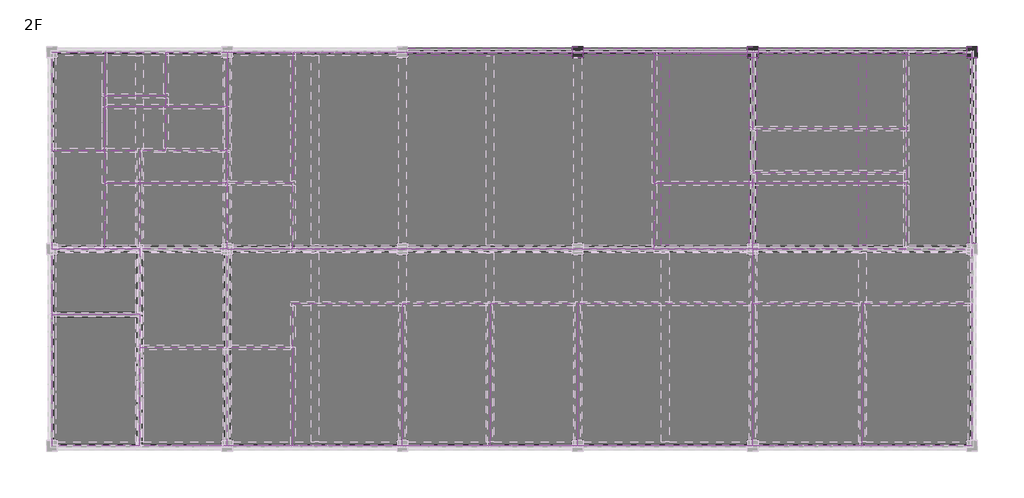
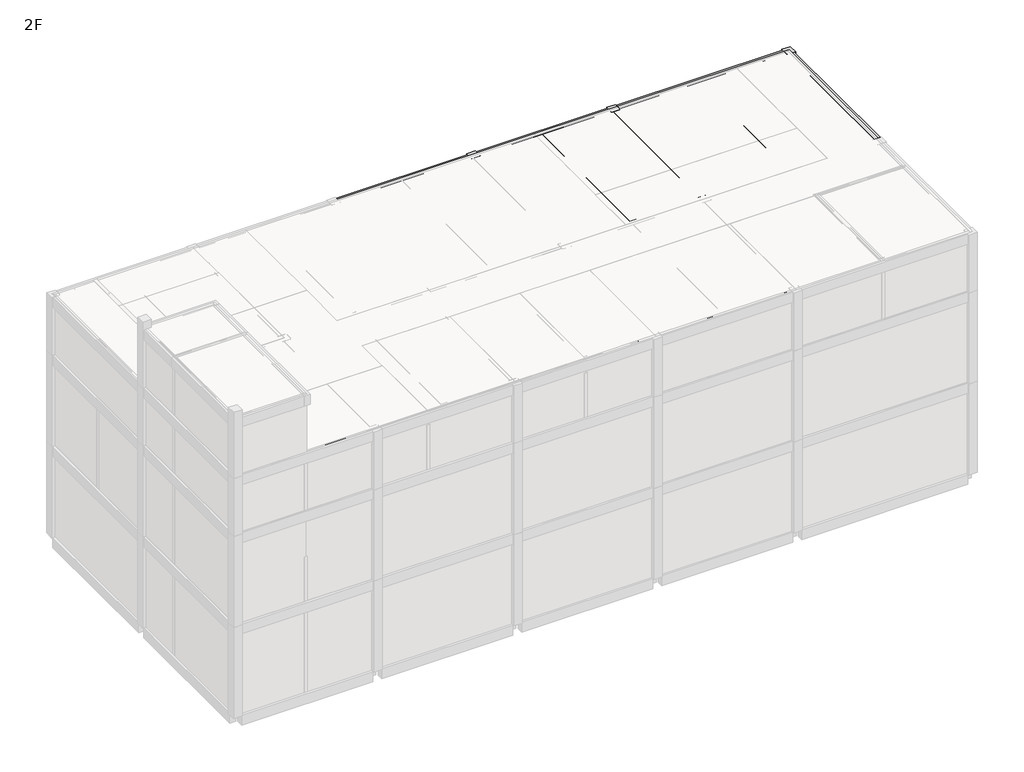
# One storey, part 7 of 7: 39 proxies, 28 beams, 9 columns.
"""IFC4 building model written with IfcOpenShell, lengths in millimetres."""

import ifcopenshell
import ifcopenshell.guid

model = None  # the IFC model being written
_history = None  # IfcOwnerHistory: only IFC2X3 demands one
_inside = {}  # id of a spatial element -> (the spatial element, [elements in it])
_under = {}  # id of a project, library or spatial element -> (it, [spatial elements below it])
_declared = {}  # id of a project -> (the project, [libraries it declares])
_typed = {}  # id of a type object -> (the type object, [elements of that type])
_made_of = {}  # id of a material, layer set ... -> (it, [elements and type objects made of it])


def new_model(schema):
    """Start an empty IFC model of exactly this schema.

    Asked for "IFC4X3", IfcOpenShell would pick the latest addendum, in which some entities
    have other attributes; the version numbers below select the first issue.
    IFC2X3 requires an IfcOwnerHistory on every rooted entity: one is made here for all.
    """
    global model, _history
    if schema == "IFC4X3":
        model = ifcopenshell.file(schema_version=(4, 3, 0, 0))
    else:
        model = ifcopenshell.file(schema=schema)
    _inside.clear()
    _under.clear()
    _declared.clear()
    _typed.clear()
    _made_of.clear()
    _history = None
    if model.schema == "IFC2X3":
        org = make("IfcOrganization", Name="unknown")
        user = make(
            "IfcPersonAndOrganization",
            ThePerson=make("IfcPerson", FamilyName="unknown"),
            TheOrganization=org,
        )
        app = make(
            "IfcApplication",
            ApplicationDeveloper=org,
            Version="unknown",
            ApplicationFullName="unknown",
            ApplicationIdentifier="unknown",
        )
        _history = make(
            "IfcOwnerHistory",
            OwningUser=user,
            OwningApplication=app,
            ChangeAction="ADDED",
            CreationDate=0,
        )
    return model


def make(cls, **values):
    """One entity of the class cls with the attributes given. An attribute that is None is left unset."""
    return model.create_entity(
        cls, **{name: value for name, value in values.items() if value is not None}
    )


def rooted(cls, **values):
    """An entity with a GlobalId (a new one), such as an element, a storey or a relation."""
    return make(cls, GlobalId=ifcopenshell.guid.new(), OwnerHistory=_history, **values)


def si_unit(unit_type, name, prefix=None):
    """IfcSIUnit, for example si_unit("LENGTHUNIT", "METRE", prefix="MILLI")."""
    return make("IfcSIUnit", UnitType=unit_type, Prefix=prefix, Name=name)


def assignment(units):
    """IfcUnitAssignment: the units of a project."""
    return None if units is None else make("IfcUnitAssignment", Units=units)


def point(xyz):
    """IfcCartesianPoint."""
    return None if xyz is None else make("IfcCartesianPoint", Coordinates=xyz)


def direction(xyz):
    """IfcDirection."""
    return None if xyz is None else make("IfcDirection", DirectionRatios=xyz)


def frame(location, z_axis=None, x_axis=None):
    """IfcAxis2Placement3D, a coordinate frame: its origin and axes. An axis left out is left unset."""
    return make(
        "IfcAxis2Placement3D",
        Location=point(location),
        Axis=direction(z_axis),
        RefDirection=direction(x_axis),
    )


def origin():
    """The frame at (0, 0, 0) with its axes left unset."""
    return frame((0.0, 0.0, 0.0))


def origin_with_axes():
    """The frame at (0, 0, 0) with the z axis (0, 0, 1) and the x axis (1, 0, 0) written out."""
    return frame((0.0, 0.0, 0.0), z_axis=(0.0, 0.0, 1.0), x_axis=(1.0, 0.0, 0.0))


def place(relative_to, where):
    """IfcLocalPlacement: puts the frame where relative to a parent placement (None: the world)."""
    return make(
        "IfcLocalPlacement", PlacementRelTo=relative_to, RelativePlacement=where
    )


def context(
    kind, dimensions, precision=None, world=None, true_north=None, identifier=None
):
    """IfcGeometricRepresentationContext, for example the 3D "Model" context."""
    return make(
        "IfcGeometricRepresentationContext",
        ContextIdentifier=identifier,
        ContextType=kind,
        CoordinateSpaceDimension=dimensions,
        Precision=precision,
        WorldCoordinateSystem=world,
        TrueNorth=true_north,
    )


def project(units=None, contexts=None):
    """IfcProject with its units and contexts."""
    return rooted(
        "IfcProject",
        Name="project",
        RepresentationContexts=contexts,
        UnitsInContext=assignment(units),
    )


def spatial(cls, under=None, at=None, **own):
    """A site, building, storey or space (cls), placed at a placement, below another one or the project."""
    s = rooted(cls, ObjectPlacement=at, **own)
    if under is not None:
        _under.setdefault(under.id(), (under, []))[1].append(s)
    return s


def polyline(points):
    """IfcPolyline through the points."""
    return make("IfcPolyline", Points=[point(p) for p in points])


def outline(outer, holes=None, kind="AREA"):
    """IfcArbitraryClosedProfileDef: a profile drawn as a closed curve; with holes, ...WithVoids."""
    if holes is None:
        return make("IfcArbitraryClosedProfileDef", ProfileType=kind, OuterCurve=outer)
    return make(
        "IfcArbitraryProfileDefWithVoids",
        ProfileType=kind,
        OuterCurve=outer,
        InnerCurves=holes,
    )


def extrude(swept, where, along, depth):
    """IfcExtrudedAreaSolid: the profile swept, set in the frame where, extruded along a direction by depth."""
    return make(
        "IfcExtrudedAreaSolid",
        SweptArea=swept,
        Position=where,
        ExtrudedDirection=direction(along),
        Depth=depth,
    )


def faces_of(points, faces, orient=None, outer=None):
    """IfcFace entities. A face is a list of loops; a loop is a list of indices into points, from 0.

    orient and outer hold one flag for each loop. By default every Orientation is true, the
    first loop of a face is its IfcFaceOuterBound and the others are IfcFaceBound.
    """
    made = []
    for i, loops in enumerate(faces):
        bounds = []
        for j, loop in enumerate(loops):
            is_outer = j == 0 if outer is None else outer[i][j]
            bounds.append(
                make(
                    "IfcFaceOuterBound" if is_outer else "IfcFaceBound",
                    Bound=make("IfcPolyLoop", Polygon=[points[k] for k in loop]),
                    Orientation=True if orient is None else orient[i][j],
                )
            )
        made.append(make("IfcFace", Bounds=bounds))
    return made


def faceted_brep(points, faces, orient=None, outer=None, voids=None):
    """IfcFacetedBrep: a solid bounded by flat faces; with voids (closed shells), ...WithVoids."""
    shared = [point(p) for p in points]
    hull = make("IfcClosedShell", CfsFaces=faces_of(shared, faces, orient, outer))
    if voids is None:
        return make("IfcFacetedBrep", Outer=hull)
    return make(
        "IfcFacetedBrepWithVoids",
        Outer=hull,
        Voids=[
            make(cls, CfsFaces=faces_of(shared, fs, o, b)) for cls, fs, o, b in voids
        ],
    )


def shape(context_of_items, identifier, shape_type, items):
    """IfcShapeRepresentation: the items that make up one representation, for example the "Body"."""
    return make(
        "IfcShapeRepresentation",
        ContextOfItems=context_of_items,
        RepresentationIdentifier=identifier,
        RepresentationType=shape_type,
        Items=items,
    )


def source(mapping_origin, context_of_items, identifier, shape_type, items):
    """IfcRepresentationMap: a shape defined once, which mapped items show again and again."""
    return make(
        "IfcRepresentationMap",
        MappingOrigin=mapping_origin,
        MappedRepresentation=shape(context_of_items, identifier, shape_type, items),
    )


def transform(
    local_origin,
    x_axis=None,
    y_axis=None,
    z_axis=None,
    scale=None,
    scale2=None,
    scale3=None,
    uniform=True,
):
    """IfcCartesianTransformationOperator3D, or its non-uniform kind. x_axis, y_axis, z_axis: its Axis1, 2, 3."""
    if uniform:
        return make(
            "IfcCartesianTransformationOperator3D",
            Axis1=direction(x_axis),
            Axis2=direction(y_axis),
            LocalOrigin=point(local_origin),
            Scale=scale,
            Axis3=direction(z_axis),
        )
    return make(
        "IfcCartesianTransformationOperator3DnonUniform",
        Axis1=direction(x_axis),
        Axis2=direction(y_axis),
        LocalOrigin=point(local_origin),
        Scale=scale,
        Axis3=direction(z_axis),
        Scale2=scale2,
        Scale3=scale3,
    )


def mapped(mapping_source, mapping_target):
    """IfcMappedItem: shows the shape of a source again, moved by a transform."""
    return make(
        "IfcMappedItem", MappingSource=mapping_source, MappingTarget=mapping_target
    )


def made_of(thing, what):
    """Note that an element or type object is made of a material, layer set ...; save() writes the relation."""
    if what is not None:
        _made_of.setdefault(what.id(), (what, []))[1].append(thing)
    return thing


def element(
    cls,
    number,
    at=None,
    inside=None,
    cuts=None,
    type_object=None,
    material=None,
    context=None,
    identifier="Body",
    shape_type=None,
    held_by="IfcProductDefinitionShape",
    body=None,
    shapes=None,
    **own,
):
    """One element of the class cls, such as IfcWall. Its Tag is "e" and its number.

    at: its placement. inside: the storey or other place that contains it. cuts: it is an
    opening in that element (IfcRelVoidsElement). A single representation is given by context,
    identifier, shape_type and body (its items); several are given by shapes. held_by: the class
    of the entity that holds the representations. save() writes the other relations.
    """
    e = rooted(cls, Tag="e%d" % number, ObjectPlacement=at, **own)
    if body is not None:
        shapes = [shape(context, identifier, shape_type, body)]
    if shapes is not None:
        e.Representation = make(held_by, Representations=shapes)
    if inside is not None:
        _inside.setdefault(inside.id(), (inside, []))[1].append(e)
    if cuts is not None:
        rooted(
            "IfcRelVoidsElement", RelatingBuildingElement=cuts, RelatedOpeningElement=e
        )
    if type_object is not None:
        _typed.setdefault(type_object.id(), (type_object, []))[1].append(e)
    return made_of(e, material)


def aggregate(whole, parts):
    """IfcRelAggregates: a whole, such as a stair, and the parts it consists of."""
    return rooted("IfcRelAggregates", RelatingObject=whole, RelatedObjects=parts)


def save(model, path):
    """Write the relations noted so far, then the file.

    IfcRelAggregates (storeys below a building ...), IfcRelContainedInSpatialStructure (elements
    in a storey), IfcRelDefinesByType, IfcRelAssociatesMaterial and IfcRelDeclares: one each for
    every whole, place, type object, material and project.
    """
    for whole, parts in _under.values():
        aggregate(whole, parts)
    for where, things in _inside.values():
        rooted(
            "IfcRelContainedInSpatialStructure",
            RelatedElements=things,
            RelatingStructure=where,
        )
    for kind, things in _typed.values():
        rooted("IfcRelDefinesByType", RelatedObjects=things, RelatingType=kind)
    for what, things in _made_of.values():
        rooted("IfcRelAssociatesMaterial", RelatedObjects=things, RelatingMaterial=what)
    for by, libraries in _declared.values():
        rooted("IfcRelDeclares", RelatingContext=by, RelatedDefinitions=libraries)
    model.write(path)


def generic_models_c89eb543(model_context):
    return source(origin(), model_context, "Body", "SweptSolid", [
        extrude(outline(polyline([(2000.0, 3000.0), (2000.0, -3000.0), (-2000.0, -3000.0), (-2000.0, 3000.0), (2000.0, 3000.0)])), origin_with_axes(), (0.0, 0.0, 1.0), 3500.0),
    ])


def generic_models_50f5a469(model_context):
    return source(origin(), model_context, "Body", "SweptSolid", [
        extrude(outline(polyline([(4500.0, 16000.0), (4500.0, -16000.0), (-4500.0, -16000.0), (-4500.0, 16000.0), (4500.0, 16000.0)])), origin_with_axes(), (0.0, 0.0, 1.0), 5500.0),
    ])


def generic_models_8b5775ea(model_context):
    return source(origin(), model_context, "Body", "SweptSolid", [
        extrude(outline(polyline([(4500.0, 17000.0), (4500.0, -17000.0), (-4500.0, -17000.0), (-4500.0, 17000.0), (4500.0, 17000.0)])), origin_with_axes(), (0.0, 0.0, 1.0), 5500.0),
    ])


def generic_models_2d265e4a(model_context):
    return source(origin(), model_context, "Body", "SweptSolid", [
        extrude(outline(polyline([(4500.0, 5000.0), (4500.0, -5000.0), (-4500.0, -5000.0), (-4500.0, 5000.0), (4500.0, 5000.0)])), origin_with_axes(), (0.0, 0.0, 1.0), 5500.0),
    ])


def generic_models_8934d72c(model_context):
    return source(origin(), model_context, "Body", "SweptSolid", [
        extrude(outline(polyline([(2000.0, 4500.0), (2000.0, -4500.0), (-2000.0, -4500.0), (-2000.0, 4500.0), (2000.0, 4500.0)])), origin_with_axes(), (0.0, 0.0, 1.0), 5500.0),
    ])


def generic_models_626d8198(model_context):
    return source(origin(), model_context, "Body", "SweptSolid", [
        extrude(outline(polyline([(2000.0, 1500.0), (2000.0, -1500.0), (-2000.0, -1500.0), (-2000.0, 1500.0), (2000.0, 1500.0)])), origin_with_axes(), (0.0, 0.0, 1.0), 5500.0),
    ])


def generic_models_cc1dae17(model_context):
    return source(origin(), model_context, "Body", "SweptSolid", [
        extrude(outline(polyline([(2000.0, 3000.0), (2000.0, -3000.0), (-2000.0, -3000.0), (-2000.0, 3000.0), (2000.0, 3000.0)])), origin_with_axes(), (0.0, 0.0, 1.0), 5500.0),
    ])


def generic_models_7ea3b148(model_context):
    return source(origin(), model_context, "Body", "SweptSolid", [
        extrude(outline(polyline([(4500.0, 12000.0), (4500.0, -12000.0), (-4500.0, -12000.0), (-4500.0, 12000.0), (4500.0, 12000.0)])), origin_with_axes(), (0.0, 0.0, 1.0), 5500.0),
    ])


def generic_models_85ff21bb(model_context):
    return source(origin(), model_context, "Body", "SweptSolid", [
        extrude(outline(polyline([(3500.0, 1750.0), (3500.0, -1750.0), (-3500.0, -1750.0), (-3500.0, 1750.0), (3500.0, 1750.0)])), origin_with_axes(), (0.0, 0.0, 1.0), 5500.0),
    ])


def generic_models_570012e4(model_context):
    return source(origin(), model_context, "Body", "SweptSolid", [
        extrude(outline(polyline([(1200.0, 2250.0), (1200.0, -2250.0), (-1200.0, -2250.0), (-1200.0, 2250.0), (1200.0, 2250.0)])), origin_with_axes(), (0.0, 0.0, 1.0), 5500.0),
    ])


def generic_models_971c0b89(model_context):
    return source(origin(), model_context, "Body", "SweptSolid", [
        extrude(outline(polyline([(2000.0, 2250.0), (2000.0, -2250.0), (-2000.0, -2250.0), (-2000.0, 2250.0), (2000.0, 2250.0)])), origin_with_axes(), (0.0, 0.0, 1.0), 5500.0),
    ])


def generic_models_ac48a1a3(model_context):
    return source(origin(), model_context, "Body", "SweptSolid", [
        extrude(outline(polyline([(1400.0, 2250.0), (1400.0, -2250.0), (-1400.0, -2250.0), (-1400.0, 2250.0), (1400.0, 2250.0)])), origin_with_axes(), (0.0, 0.0, 1.0), 5500.0),
    ])


def generic_models_ee32b0c6(model_context):
    return source(origin(), model_context, "Body", "SweptSolid", [
        extrude(outline(polyline([(1400.0, 1000.0), (1400.0, -1000.0), (-1400.0, -1000.0), (-1400.0, 1000.0), (1400.0, 1000.0)])), origin_with_axes(), (0.0, 0.0, 1.0), 5500.0),
    ])


def generic_models_0ee3397c(model_context):
    return source(origin(), model_context, "Body", "SweptSolid", [
        extrude(outline(polyline([(1400.0, 1250.0), (1400.0, -1250.0), (-1400.0, -1250.0), (-1400.0, 1250.0), (1400.0, 1250.0)])), origin_with_axes(), (0.0, 0.0, 1.0), 5500.0),
    ])


def generic_models_8c4134a9(model_context):
    return source(origin(), model_context, "Body", "SweptSolid", [
        extrude(outline(polyline([(3250.0, 2000.0), (3250.0, -2000.0), (-3250.0, -2000.0), (-3250.0, 2000.0), (3250.0, 2000.0)])), origin_with_axes(), (0.0, 0.0, 1.0), 3500.0),
    ])


def generic_models_ccc8c8c2(model_context):
    return source(origin(), model_context, "Body", "SweptSolid", [
        extrude(outline(polyline([(3000.0, 5750.0), (3000.0, -5750.0), (-3000.0, -5750.0), (-3000.0, 5750.0), (3000.0, 5750.0)])), origin_with_axes(), (0.0, 0.0, 1.0), 3500.0),
    ])


def generic_models_70f6ae48(model_context):
    return source(origin(), model_context, "Body", "SweptSolid", [
        extrude(outline(polyline([(3250.0, 4000.0), (3250.0, -4000.0), (-3250.0, -4000.0), (-3250.0, 4000.0), (3250.0, 4000.0)])), origin_with_axes(), (0.0, 0.0, 1.0), 3500.0),
    ])


def generic_models_f0561c1d(model_context):
    return source(origin(), model_context, "Body", "SweptSolid", [
        extrude(outline(polyline([(4500.0, 8250.0), (4500.0, -8250.0), (-4500.0, -8250.0), (-4500.0, 8250.0), (4500.0, 8250.0)])), origin_with_axes(), (0.0, 0.0, 1.0), 3500.0),
    ])


def generic_models_249c6621(model_context):
    return source(origin(), model_context, "Body", "SweptSolid", [
        extrude(outline(polyline([(3250.0, 2500.0), (3250.0, -2500.0), (-3250.0, -2500.0), (-3250.0, 2500.0), (3250.0, 2500.0)])), origin_with_axes(), (0.0, 0.0, 1.0), 3500.0),
    ])


def generic_models_f1f4091a(model_context):
    return source(origin(), model_context, "Body", "SweptSolid", [
        extrude(outline(polyline([(1500.0, 5750.0), (1500.0, -5750.0), (-1500.0, -5750.0), (-1500.0, 5750.0), (1500.0, 5750.0)])), origin_with_axes(), (0.0, 0.0, 1.0), 3500.0),
    ])


def generic_models_10b6925f(model_context):
    return source(origin(), model_context, "Body", "SweptSolid", [
        extrude(outline(polyline([(2250.0, 3500.0), (2250.0, -3500.0), (-2250.0, -3500.0), (-2250.0, 3500.0), (2250.0, 3500.0)])), origin_with_axes(), (0.0, 0.0, 1.0), 3500.0),
    ])


def generic_models_b37916ea(model_context):
    return source(origin(), model_context, "Body", "SweptSolid", [
        extrude(outline(polyline([(1750.0, 2800.0), (1750.0, -2800.0), (-1750.0, -2800.0), (-1750.0, 2800.0), (1750.0, 2800.0)])), origin_with_axes(), (0.0, 0.0, 1.0), 3500.0),
    ])


def generic_models_6c75c912(model_context):
    return source(origin(), model_context, "Body", "SweptSolid", [
        extrude(outline(polyline([(1250.0, 2800.0), (1250.0, -2800.0), (-1250.0, -2800.0), (-1250.0, 2800.0), (1250.0, 2800.0)])), origin_with_axes(), (0.0, 0.0, 1.0), 3500.0),
    ])


def generic_models_a5818909(model_context):
    return source(origin(), model_context, "Body", "SweptSolid", [
        extrude(outline(polyline([(3000.0, 1500.0), (3000.0, -1500.0), (-3000.0, -1500.0), (-3000.0, 1500.0), (3000.0, 1500.0)])), origin_with_axes(), (0.0, 0.0, 1.0), 3500.0),
    ])


def generic_models_f42d0df8(model_context):
    return source(origin(), model_context, "Body", "SweptSolid", [
        extrude(outline(polyline([(1500.0, 2800.0), (1500.0, -2800.0), (-1500.0, -2800.0), (-1500.0, 2800.0), (1500.0, 2800.0)])), origin_with_axes(), (0.0, 0.0, 1.0), 3500.0),
    ])


def generic_models_3f6e5246(model_context):
    return source(origin(), model_context, "Body", "SweptSolid", [
        extrude(outline(polyline([(1200.0, 4500.0), (1200.0, -4500.0), (-1200.0, -4500.0), (-1200.0, 4500.0), (1200.0, 4500.0)])), origin_with_axes(), (0.0, 0.0, 1.0), 3500.0),
    ])


def generic_models_4c644d41(model_context):
    return source(origin(), model_context, "Body", "SweptSolid", [
        extrude(outline(polyline([(2000.0, 1500.0), (2000.0, -1500.0), (-2000.0, -1500.0), (-2000.0, 1500.0), (2000.0, 1500.0)])), origin_with_axes(), (0.0, 0.0, 1.0), 3500.0),
    ])


def generic_models_3d03af35(model_context):
    return source(origin(), model_context, "Body", "SweptSolid", [
        extrude(outline(polyline([(21000.0, 9000.0), (21000.0, -9000.0), (-21000.0, -9000.0), (-21000.0, 9000.0), (21000.0, 9000.0)])), origin_with_axes(), (0.0, 0.0, 1.0), 5500.0),
    ])


def generic_models_bb515c93(model_context):
    return source(origin(), model_context, "Body", "SweptSolid", [
        extrude(outline(polyline([(9000.0, 21000.0), (9000.0, -21000.0), (-9000.0, -21000.0), (-9000.0, 21000.0), (9000.0, 21000.0)])), origin_with_axes(), (0.0, 0.0, 1.0), 3500.0),
    ])


model = new_model("IFC4")

# Units and contexts
model_context = context("Model", 3, world=origin())
ifc_project = project(units=[si_unit("LENGTHUNIT", "METRE", prefix="MILLI")], contexts=[model_context])

# Site, building, storey
site = spatial("IfcSite", under=ifc_project)
building = spatial("IfcBuilding", under=site)
storey = spatial("IfcBuildingStorey", under=building, Name="2F", Elevation=3500.0)

# Beams
placement = place(None, origin())
element("IfcBeam", 1, ObjectType="Concrete-Rectangular-Beam : BM111_400x500_RG1", at=placement, inside=storey, context=model_context, shape_type="SweptSolid", body=[
    extrude(outline(polyline([(73634.6521483, 173098.8614395), (73284.6521483, 173098.8614395), (73284.6521483, 181748.8614395), (73634.6521483, 181748.8614395), (73634.6521483, 173098.8614395)])), frame((0.0, 0.0, 2900.0), z_axis=(0.0, 0.0, 1.0), x_axis=(1.0, 0.0, 0.0)), (0.0, 0.0, 1.0), 600.0),
])
element("IfcBeam", 2, ObjectType="Concrete-Rectangular-Beam : BM111_400x500_RG1", at=placement, inside=storey, context=model_context, shape_type="SweptSolid", body=[
    extrude(outline(polyline([(82634.6521483, 173098.8614395), (82284.6521483, 173098.8614395), (82284.6521483, 181748.8614395), (82634.6521483, 181748.8614395), (82634.6521483, 173098.8614395)])), frame((0.0, 0.0, 2900.0), z_axis=(0.0, 0.0, 1.0), x_axis=(1.0, 0.0, 0.0)), (0.0, 0.0, 1.0), 600.0),
])
element("IfcBeam", 3, ObjectType="Concrete-Rectangular-Beam : BM111_400x500_RG1", at=placement, inside=storey, context=model_context, shape_type="SweptSolid", body=[
    extrude(outline(polyline([(73634.6521483, 173098.8614395), (73284.6521483, 173098.8614395), (73284.6521483, 181748.8614395), (73634.6521483, 181748.8614395), (73634.6521483, 173098.8614395)])), frame((0.0, 0.0, 8400.0), z_axis=(0.0, 0.0, 1.0), x_axis=(1.0, 0.0, 0.0)), (0.0, 0.0, 1.0), 600.0),
])
element("IfcBeam", 4, ObjectType="Concrete-Rectangular-Beam : BM111_400x500_RG1", at=placement, inside=storey, context=model_context, shape_type="SweptSolid", body=[
    extrude(outline(polyline([(82634.6521483, 173098.8614395), (82284.6521483, 173098.8614395), (82284.6521483, 181748.8614395), (82634.6521483, 181748.8614395), (82634.6521483, 173098.8614395)])), frame((0.0, 0.0, 8400.0), z_axis=(0.0, 0.0, 1.0), x_axis=(1.0, 0.0, 0.0)), (0.0, 0.0, 1.0), 600.0),
])
element("IfcBeam", 5, ObjectType="Concrete-Rectangular-Beam : BM111_400x500_RG1", at=placement, inside=storey, context=model_context, shape_type="SweptSolid", body=[
    extrude(outline(polyline([(73634.6521483, 173098.8614395), (73284.6521483, 173098.8614395), (73284.6521483, 181748.8614395), (73634.6521483, 181748.8614395), (73634.6521483, 173098.8614395)])), frame((0.0, 0.0, 13900.0), z_axis=(0.0, 0.0, 1.0), x_axis=(1.0, 0.0, 0.0)), (0.0, 0.0, 1.0), 600.0),
])
element("IfcBeam", 6, ObjectType="Concrete-Rectangular-Beam : BM111_400x500_RG1", at=placement, inside=storey, context=model_context, shape_type="SweptSolid", body=[
    extrude(outline(polyline([(82634.6521483, 173098.8614395), (82284.6521483, 173098.8614395), (82284.6521483, 181748.8614395), (82634.6521483, 181748.8614395), (82634.6521483, 173098.8614395)])), frame((0.0, 0.0, 13900.0), z_axis=(0.0, 0.0, 1.0), x_axis=(1.0, 0.0, 0.0)), (0.0, 0.0, 1.0), 600.0),
])
element("IfcBeam", 7, ObjectType="Concrete-Rectangular-Beam : BM111_400x500_RG1", at=placement, inside=storey, context=model_context, shape_type="SweptSolid", body=[
    extrude(outline(polyline([(73634.6521483, 173098.8614395), (73284.6521483, 173098.8614395), (73284.6521483, 181748.8614395), (73634.6521483, 181748.8614395), (73634.6521483, 173098.8614395)])), frame((0.0, 0.0, 17400.0), z_axis=(0.0, 0.0, 1.0), x_axis=(1.0, 0.0, 0.0)), (0.0, 0.0, 1.0), 600.0),
])
element("IfcBeam", 8, ObjectType="Concrete-Rectangular-Beam : BM111_400x500_RG1", at=placement, inside=storey, context=model_context, shape_type="SweptSolid", body=[
    extrude(outline(polyline([(82634.6521483, 173098.8614395), (82284.6521483, 173098.8614395), (82284.6521483, 181748.8614395), (82634.6521483, 181748.8614395), (82634.6521483, 173098.8614395)])), frame((0.0, 0.0, 17400.0), z_axis=(0.0, 0.0, 1.0), x_axis=(1.0, 0.0, 0.0)), (0.0, 0.0, 1.0), 600.0),
])
element("IfcBeam", 9, ObjectType="Concrete-Rectangular-Beam : BM111_400x500_RG1", at=placement, inside=storey, context=model_context, shape_type="Brep", body=[
    faceted_brep([(61709.6521483, 182098.8614395, 3500.0), (61709.6521483, 181748.8614395, 3500.0), (65284.6521483, 181748.8614395, 3500.0), (65634.6521483, 181748.8614395, 3500.0), (69209.6521483, 181748.8614395, 3500.0), (69209.6521483, 182098.8614395, 3500.0), (61709.6521483, 181748.8614395, 2900.0), (65284.6521483, 181748.8614395, 2900.0), (65634.6521483, 181748.8614395, 2900.0), (69209.6521483, 181748.8614395, 2900.0), (61709.6521483, 182098.8614395, 2900.0), (69209.6521483, 182098.8614395, 2900.0)], [[[0, 1, 2, 3, 4, 5]], [[1, 6, 7, 8, 9, 4, 3, 2]], [[6, 10, 11, 9, 8, 7]], [[10, 0, 5, 11]], [[1, 0, 10, 6]], [[5, 4, 9, 11]]]),
])
element("IfcBeam", 10, ObjectType="Concrete-Rectangular-Beam : BM111_400x500_RG1", at=placement, inside=storey, context=model_context, shape_type="Brep", body=[
    faceted_brep([(69709.6521483, 182098.8614395, 3500.0), (69709.6521483, 181748.8614395, 3500.0), (73284.6521483, 181748.8614395, 3500.0), (73634.6521483, 181748.8614395, 3500.0), (77209.6521483, 181748.8614395, 3500.0), (77209.6521483, 182098.8614395, 3500.0), (69709.6521483, 181748.8614395, 2900.0), (73284.6521483, 181748.8614395, 2900.0), (73634.6521483, 181748.8614395, 2900.0), (77209.6521483, 181748.8614395, 2900.0), (69709.6521483, 182098.8614395, 2900.0), (77209.6521483, 182098.8614395, 2900.0)], [[[0, 1, 2, 3, 4, 5]], [[1, 6, 7, 8, 9, 4, 3, 2]], [[6, 10, 11, 9, 8, 7]], [[10, 0, 5, 11]], [[1, 0, 10, 6]], [[5, 4, 9, 11]]]),
])
element("IfcBeam", 11, ObjectType="Concrete-Rectangular-Beam : BM111_400x500_RG1", at=placement, inside=storey, context=model_context, shape_type="Brep", body=[
    faceted_brep([(77709.6521483, 182098.8614395, 3500.0), (77709.6521483, 181748.8614395, 3500.0), (82284.6521483, 181748.8614395, 3500.0), (82634.6521483, 181748.8614395, 3500.0), (87209.6521483, 181748.8614395, 3500.0), (87209.6521483, 182098.8614395, 3500.0), (77709.6521483, 181748.8614395, 2900.0), (82284.6521483, 181748.8614395, 2900.0), (82634.6521483, 181748.8614395, 2900.0), (87209.6521483, 181748.8614395, 2900.0), (77709.6521483, 182098.8614395, 2900.0), (87209.6521483, 182098.8614395, 2900.0)], [[[0, 1, 2, 3, 4, 5]], [[1, 6, 7, 8, 9, 4, 3, 2]], [[6, 10, 11, 9, 8, 7]], [[10, 0, 5, 11]], [[1, 0, 10, 6]], [[5, 4, 9, 11]]]),
])
element("IfcBeam", 12, ObjectType="Concrete-Rectangular-Beam : BM111_400x500_RG1", at=placement, inside=storey, context=model_context, shape_type="Brep", body=[
    faceted_brep([(61709.6521483, 182098.8614395, 9000.0), (61709.6521483, 181748.8614395, 9000.0), (65284.6521483, 181748.8614395, 9000.0), (65634.6521483, 181748.8614395, 9000.0), (69209.6521483, 181748.8614395, 9000.0), (69209.6521483, 182098.8614395, 9000.0), (61709.6521483, 181748.8614395, 8400.0), (65284.6521483, 181748.8614395, 8400.0), (65634.6521483, 181748.8614395, 8400.0), (69209.6521483, 181748.8614395, 8400.0), (61709.6521483, 182098.8614395, 8400.0), (69209.6521483, 182098.8614395, 8400.0)], [[[0, 1, 2, 3, 4, 5]], [[1, 6, 7, 8, 9, 4, 3, 2]], [[6, 10, 11, 9, 8, 7]], [[10, 0, 5, 11]], [[1, 0, 10, 6]], [[5, 4, 9, 11]]]),
])
element("IfcBeam", 13, ObjectType="Concrete-Rectangular-Beam : BM111_400x500_RG1", at=placement, inside=storey, context=model_context, shape_type="Brep", body=[
    faceted_brep([(69709.6521483, 182098.8614395, 9000.0), (69709.6521483, 181748.8614395, 9000.0), (73284.6521483, 181748.8614395, 9000.0), (73634.6521483, 181748.8614395, 9000.0), (77209.6521483, 181748.8614395, 9000.0), (77209.6521483, 182098.8614395, 9000.0), (69709.6521483, 181748.8614395, 8400.0), (73284.6521483, 181748.8614395, 8400.0), (73634.6521483, 181748.8614395, 8400.0), (77209.6521483, 181748.8614395, 8400.0), (69709.6521483, 182098.8614395, 8400.0), (77209.6521483, 182098.8614395, 8400.0)], [[[0, 1, 2, 3, 4, 5]], [[1, 6, 7, 8, 9, 4, 3, 2]], [[6, 10, 11, 9, 8, 7]], [[10, 0, 5, 11]], [[1, 0, 10, 6]], [[5, 4, 9, 11]]]),
])
element("IfcBeam", 14, ObjectType="Concrete-Rectangular-Beam : BM111_400x500_RG1", at=placement, inside=storey, context=model_context, shape_type="Brep", body=[
    faceted_brep([(77709.6521483, 182098.8614395, 9000.0), (77709.6521483, 181748.8614395, 9000.0), (82284.6521483, 181748.8614395, 9000.0), (82634.6521483, 181748.8614395, 9000.0), (87209.6521483, 181748.8614395, 9000.0), (87209.6521483, 182098.8614395, 9000.0), (77709.6521483, 181748.8614395, 8400.0), (82284.6521483, 181748.8614395, 8400.0), (82634.6521483, 181748.8614395, 8400.0), (87209.6521483, 181748.8614395, 8400.0), (77709.6521483, 182098.8614395, 8400.0), (87209.6521483, 182098.8614395, 8400.0)], [[[0, 1, 2, 3, 4, 5]], [[1, 6, 7, 8, 9, 4, 3, 2]], [[6, 10, 11, 9, 8, 7]], [[10, 0, 5, 11]], [[1, 0, 10, 6]], [[5, 4, 9, 11]]]),
])
element("IfcBeam", 15, ObjectType="Concrete-Rectangular-Beam : BM111_400x500_RG1", at=placement, inside=storey, context=model_context, shape_type="Brep", body=[
    faceted_brep([(61709.6521483, 182098.8614395, 14500.0), (61709.6521483, 181748.8614395, 14500.0), (65284.6521483, 181748.8614395, 14500.0), (65634.6521483, 181748.8614395, 14500.0), (69209.6521483, 181748.8614395, 14500.0), (69209.6521483, 182098.8614395, 14500.0), (61709.6521483, 181748.8614395, 13900.0), (65284.6521483, 181748.8614395, 13900.0), (65634.6521483, 181748.8614395, 13900.0), (69209.6521483, 181748.8614395, 13900.0), (61709.6521483, 182098.8614395, 13900.0), (69209.6521483, 182098.8614395, 13900.0)], [[[0, 1, 2, 3, 4, 5]], [[1, 6, 7, 8, 9, 4, 3, 2]], [[6, 10, 11, 9, 8, 7]], [[10, 0, 5, 11]], [[1, 0, 10, 6]], [[5, 4, 9, 11]]]),
])
element("IfcBeam", 16, ObjectType="Concrete-Rectangular-Beam : BM111_400x500_RG1", at=placement, inside=storey, context=model_context, shape_type="Brep", body=[
    faceted_brep([(69709.6521483, 182098.8614395, 14500.0), (69709.6521483, 181748.8614395, 14500.0), (73284.6521483, 181748.8614395, 14500.0), (73634.6521483, 181748.8614395, 14500.0), (77209.6521483, 181748.8614395, 14500.0), (77209.6521483, 182098.8614395, 14500.0), (69709.6521483, 181748.8614395, 13900.0), (73284.6521483, 181748.8614395, 13900.0), (73634.6521483, 181748.8614395, 13900.0), (77209.6521483, 181748.8614395, 13900.0), (69709.6521483, 182098.8614395, 13900.0), (77209.6521483, 182098.8614395, 13900.0)], [[[0, 1, 2, 3, 4, 5]], [[1, 6, 7, 8, 9, 4, 3, 2]], [[6, 10, 11, 9, 8, 7]], [[10, 0, 5, 11]], [[1, 0, 10, 6]], [[5, 4, 9, 11]]]),
])
element("IfcBeam", 17, ObjectType="Concrete-Rectangular-Beam : BM111_400x500_RG1", at=placement, inside=storey, context=model_context, shape_type="Brep", body=[
    faceted_brep([(77709.6521483, 182098.8614395, 14500.0), (77709.6521483, 181748.8614395, 14500.0), (82284.6521483, 181748.8614395, 14500.0), (82634.6521483, 181748.8614395, 14500.0), (87209.6521483, 181748.8614395, 14500.0), (87209.6521483, 182098.8614395, 14500.0), (77709.6521483, 181748.8614395, 13900.0), (82284.6521483, 181748.8614395, 13900.0), (82634.6521483, 181748.8614395, 13900.0), (87209.6521483, 181748.8614395, 13900.0), (77709.6521483, 182098.8614395, 13900.0), (87209.6521483, 182098.8614395, 13900.0)], [[[0, 1, 2, 3, 4, 5]], [[1, 6, 7, 8, 9, 4, 3, 2]], [[6, 10, 11, 9, 8, 7]], [[10, 0, 5, 11]], [[1, 0, 10, 6]], [[5, 4, 9, 11]]]),
])
element("IfcBeam", 18, ObjectType="Concrete-Rectangular-Beam : BM111_400x500_RG1", at=placement, inside=storey, context=model_context, shape_type="Brep", body=[
    faceted_brep([(61709.6521483, 182098.8614395, 18000.0), (61709.6521483, 181748.8614395, 18000.0), (65284.6521483, 181748.8614395, 18000.0), (65634.6521483, 181748.8614395, 18000.0), (69209.6521483, 181748.8614395, 18000.0), (69209.6521483, 182098.8614395, 18000.0), (61709.6521483, 181748.8614395, 17400.0), (65284.6521483, 181748.8614395, 17400.0), (65634.6521483, 181748.8614395, 17400.0), (69209.6521483, 181748.8614395, 17400.0), (61709.6521483, 182098.8614395, 17400.0), (69209.6521483, 182098.8614395, 17400.0)], [[[0, 1, 2, 3, 4, 5]], [[1, 6, 7, 8, 9, 4, 3, 2]], [[6, 10, 11, 9, 8, 7]], [[10, 0, 5, 11]], [[1, 0, 10, 6]], [[5, 4, 9, 11]]]),
])
element("IfcBeam", 19, ObjectType="Concrete-Rectangular-Beam : BM111_400x500_RG1", at=placement, inside=storey, context=model_context, shape_type="Brep", body=[
    faceted_brep([(69709.6521483, 182098.8614395, 18000.0), (69709.6521483, 181748.8614395, 18000.0), (73284.6521483, 181748.8614395, 18000.0), (73634.6521483, 181748.8614395, 18000.0), (77209.6521483, 181748.8614395, 18000.0), (77209.6521483, 182098.8614395, 18000.0), (69709.6521483, 181748.8614395, 17400.0), (73284.6521483, 181748.8614395, 17400.0), (73634.6521483, 181748.8614395, 17400.0), (77209.6521483, 181748.8614395, 17400.0), (69709.6521483, 182098.8614395, 17400.0), (77209.6521483, 182098.8614395, 17400.0)], [[[0, 1, 2, 3, 4, 5]], [[1, 6, 7, 8, 9, 4, 3, 2]], [[6, 10, 11, 9, 8, 7]], [[10, 0, 5, 11]], [[1, 0, 10, 6]], [[5, 4, 9, 11]]]),
])
element("IfcBeam", 20, ObjectType="Concrete-Rectangular-Beam : BM111_400x500_RG1", at=placement, inside=storey, context=model_context, shape_type="Brep", body=[
    faceted_brep([(77709.6521483, 182098.8614395, 18000.0), (77709.6521483, 181748.8614395, 18000.0), (82284.6521483, 181748.8614395, 18000.0), (82634.6521483, 181748.8614395, 18000.0), (87209.6521483, 181748.8614395, 18000.0), (87209.6521483, 182098.8614395, 18000.0), (77709.6521483, 181748.8614395, 17400.0), (82284.6521483, 181748.8614395, 17400.0), (82634.6521483, 181748.8614395, 17400.0), (87209.6521483, 181748.8614395, 17400.0), (77709.6521483, 182098.8614395, 17400.0), (87209.6521483, 182098.8614395, 17400.0)], [[[0, 1, 2, 3, 4, 5]], [[1, 6, 7, 8, 9, 4, 3, 2]], [[6, 10, 11, 9, 8, 7]], [[10, 0, 5, 11]], [[1, 0, 10, 6]], [[5, 4, 9, 11]]]),
])
element("IfcBeam", 21, ObjectType="Concrete-Rectangular-Beam : BM111_400x500_RG1", at=placement, inside=storey, context=model_context, shape_type="SweptSolid", body=[
    extrude(outline(polyline([(77284.6521483, 181673.8614395), (77634.6521483, 181673.8614395), (77634.6521483, 173173.8614395), (77284.6521483, 173173.8614395), (77284.6521483, 181673.8614395)])), frame((0.0, 0.0, 2900.0), z_axis=(0.0, 0.0, 1.0), x_axis=(1.0, 0.0, 0.0)), (0.0, 0.0, 1.0), 600.0),
])
element("IfcBeam", 22, ObjectType="Concrete-Rectangular-Beam : BM111_400x500_RG1", at=placement, inside=storey, context=model_context, shape_type="SweptSolid", body=[
    extrude(outline(polyline([(87284.6521483, 181673.8614395), (87634.6521483, 181673.8614395), (87634.6521483, 173173.8614395), (87284.6521483, 173173.8614395), (87284.6521483, 181673.8614395)])), frame((0.0, 0.0, 2900.0), z_axis=(0.0, 0.0, 1.0), x_axis=(1.0, 0.0, 0.0)), (0.0, 0.0, 1.0), 600.0),
])
element("IfcBeam", 23, ObjectType="Concrete-Rectangular-Beam : BM111_400x500_RG1", at=placement, inside=storey, context=model_context, shape_type="SweptSolid", body=[
    extrude(outline(polyline([(77284.6521483, 181673.8614395), (77634.6521483, 181673.8614395), (77634.6521483, 173173.8614395), (77284.6521483, 173173.8614395), (77284.6521483, 181673.8614395)])), frame((0.0, 0.0, 8400.0), z_axis=(0.0, 0.0, 1.0), x_axis=(1.0, 0.0, 0.0)), (0.0, 0.0, 1.0), 600.0),
])
element("IfcBeam", 24, ObjectType="Concrete-Rectangular-Beam : BM111_400x500_RG1", at=placement, inside=storey, context=model_context, shape_type="SweptSolid", body=[
    extrude(outline(polyline([(87284.6521483, 181673.8614395), (87634.6521483, 181673.8614395), (87634.6521483, 173173.8614395), (87284.6521483, 173173.8614395), (87284.6521483, 181673.8614395)])), frame((0.0, 0.0, 8400.0), z_axis=(0.0, 0.0, 1.0), x_axis=(1.0, 0.0, 0.0)), (0.0, 0.0, 1.0), 600.0),
])
element("IfcBeam", 25, ObjectType="Concrete-Rectangular-Beam : BM111_400x500_RG1", at=placement, inside=storey, context=model_context, shape_type="SweptSolid", body=[
    extrude(outline(polyline([(77284.6521483, 181673.8614395), (77634.6521483, 181673.8614395), (77634.6521483, 173173.8614395), (77284.6521483, 173173.8614395), (77284.6521483, 181673.8614395)])), frame((0.0, 0.0, 13900.0), z_axis=(0.0, 0.0, 1.0), x_axis=(1.0, 0.0, 0.0)), (0.0, 0.0, 1.0), 600.0),
])
element("IfcBeam", 26, ObjectType="Concrete-Rectangular-Beam : BM111_400x500_RG1", at=placement, inside=storey, context=model_context, shape_type="SweptSolid", body=[
    extrude(outline(polyline([(87284.6521483, 181673.8614395), (87634.6521483, 181673.8614395), (87634.6521483, 173173.8614395), (87284.6521483, 173173.8614395), (87284.6521483, 181673.8614395)])), frame((0.0, 0.0, 13900.0), z_axis=(0.0, 0.0, 1.0), x_axis=(1.0, 0.0, 0.0)), (0.0, 0.0, 1.0), 600.0),
])
element("IfcBeam", 27, ObjectType="Concrete-Rectangular-Beam : BM111_400x500_RG1", at=placement, inside=storey, context=model_context, shape_type="SweptSolid", body=[
    extrude(outline(polyline([(77284.6521483, 181673.8614395), (77634.6521483, 181673.8614395), (77634.6521483, 173173.8614395), (77284.6521483, 173173.8614395), (77284.6521483, 181673.8614395)])), frame((0.0, 0.0, 17400.0), z_axis=(0.0, 0.0, 1.0), x_axis=(1.0, 0.0, 0.0)), (0.0, 0.0, 1.0), 600.0),
])
element("IfcBeam", 28, ObjectType="Concrete-Rectangular-Beam : BM111_400x500_RG1", at=placement, inside=storey, context=model_context, shape_type="SweptSolid", body=[
    extrude(outline(polyline([(87284.6521483, 181673.8614395), (87634.6521483, 181673.8614395), (87634.6521483, 173173.8614395), (87284.6521483, 173173.8614395), (87284.6521483, 181673.8614395)])), frame((0.0, 0.0, 17400.0), z_axis=(0.0, 0.0, 1.0), x_axis=(1.0, 0.0, 0.0)), (0.0, 0.0, 1.0), 600.0),
])

# Proxies
generic_models_shape = generic_models_c89eb543(model_context)
element("IfcBuildingElementProxy", 29, Name="Generic Models", at=placement, inside=storey, context=model_context, shape_type="MappedRepresentation", body=[
    mapped(generic_models_shape, transform((47459.6521483, 166923.8614395, 14500.0), x_axis=(1.0, 0.0, 0.0), y_axis=(0.0, 1.0, 0.0), z_axis=(0.0, 0.0, 1.0))),
])
element("IfcBuildingElementProxy", 30, Name="Generic Models", at=placement, inside=storey, context=model_context, shape_type="MappedRepresentation", body=[
    mapped(generic_models_shape, transform((47459.6521483, 166923.8614395, 18000.0), x_axis=(1.0, 0.0, 0.0), y_axis=(0.0, 1.0, 0.0), z_axis=(0.0, 0.0, 1.0))),
])
generic_models_2_shape = generic_models_50f5a469(model_context)
element("IfcBuildingElementProxy", 31, Name="Generic Models", at=placement, inside=storey, context=model_context, shape_type="MappedRepresentation", body=[
    mapped(generic_models_2_shape, transform((61459.6521483, 177423.8614395, 3500.0), x_axis=(0.0, 1.0, 0.0), y_axis=(-1.0, 0.0, 0.0), z_axis=(0.0, 0.0, 1.0))),
])
generic_models_3_shape = generic_models_8b5775ea(model_context)
element("IfcBuildingElementProxy", 32, Name="Generic Models", at=placement, inside=storey, context=model_context, shape_type="MappedRepresentation", body=[
    mapped(generic_models_3_shape, transform((70459.6521483, 168423.8614395, 3500.0), x_axis=(0.0, 1.0, 0.0), y_axis=(-1.0, 0.0, 0.0), z_axis=(0.0, 0.0, 1.0))),
])
generic_models_4_shape = generic_models_2d265e4a(model_context)
element("IfcBuildingElementProxy", 33, Name="Generic Models", at=placement, inside=storey, context=model_context, shape_type="MappedRepresentation", body=[
    mapped(generic_models_4_shape, transform((82459.6521483, 177423.8614395, 3500.0), x_axis=(0.0, 1.0, 0.0), y_axis=(-1.0, 0.0, 0.0), z_axis=(0.0, 0.0, 1.0))),
])
generic_models_5_shape = generic_models_8934d72c(model_context)
element("IfcBuildingElementProxy", 34, Name="Generic Models", at=placement, inside=storey, context=model_context, shape_type="MappedRepresentation", body=[
    mapped(generic_models_5_shape, transform((51459.6521483, 168423.8614395, 3500.0), x_axis=(1.0, 0.0, 0.0), y_axis=(0.0, 1.0, 0.0), z_axis=(0.0, 0.0, 1.0))),
])
generic_models_6_shape = generic_models_626d8198(model_context)
element("IfcBuildingElementProxy", 35, Name="Generic Models", at=placement, inside=storey, context=model_context, shape_type="MappedRepresentation", body=[
    mapped(generic_models_6_shape, transform((47459.6521483, 171423.8614395, 3500.0), x_axis=(1.0, 0.0, 0.0), y_axis=(0.0, 1.0, 0.0), z_axis=(0.0, 0.0, 1.0))),
])
element("IfcBuildingElementProxy", 36, Name="Generic Models", at=placement, inside=storey, context=model_context, shape_type="MappedRepresentation", body=[
    mapped(generic_models_6_shape, transform((47459.6521483, 171423.8614395, 9000.0), x_axis=(1.0, 0.0, 0.0), y_axis=(0.0, 1.0, 0.0), z_axis=(0.0, 0.0, 1.0))),
])
generic_models_7_shape = generic_models_cc1dae17(model_context)
element("IfcBuildingElementProxy", 37, Name="Generic Models", at=placement, inside=storey, context=model_context, shape_type="MappedRepresentation", body=[
    mapped(generic_models_7_shape, transform((47459.6521483, 166923.8614395, 3500.0), x_axis=(1.0, 0.0, 0.0), y_axis=(0.0, 1.0, 0.0), z_axis=(0.0, 0.0, 1.0))),
])
element("IfcBuildingElementProxy", 38, Name="Generic Models", at=placement, inside=storey, context=model_context, shape_type="MappedRepresentation", body=[
    mapped(generic_models_7_shape, transform((47459.6521483, 166923.8614395, 9000.0), x_axis=(1.0, 0.0, 0.0), y_axis=(0.0, 1.0, 0.0), z_axis=(0.0, 0.0, 1.0))),
])
generic_models_8_shape = generic_models_7ea3b148(model_context)
element("IfcBuildingElementProxy", 39, Name="Generic Models", at=placement, inside=storey, context=model_context, shape_type="MappedRepresentation", body=[
    mapped(generic_models_8_shape, transform((65459.6521483, 177423.8614395, 9000.0), x_axis=(0.0, -1.0, 0.0), y_axis=(1.0, 0.0, 0.0), z_axis=(0.0, 0.0, 1.0))),
])
element("IfcBuildingElementProxy", 40, Name="Generic Models", at=placement, inside=storey, context=model_context, shape_type="MappedRepresentation", body=[
    mapped(generic_models_8_shape, transform((65459.6521483, 168423.8614395, 9000.0), x_axis=(0.0, -1.0, 0.0), y_axis=(1.0, 0.0, 0.0), z_axis=(0.0, 0.0, 1.0))),
])
generic_models_9_shape = generic_models_85ff21bb(model_context)
element("IfcBuildingElementProxy", 41, Name="Generic Models", at=placement, inside=storey, context=model_context, shape_type="MappedRepresentation", body=[
    mapped(generic_models_9_shape, transform((80959.6521483, 180173.8614395, 9000.0), x_axis=(1.0, 0.0, 0.0), y_axis=(0.0, 1.0, 0.0), z_axis=(0.0, 0.0, 1.0))),
])
element("IfcBuildingElementProxy", 42, Name="Generic Models", at=placement, inside=storey, context=model_context, shape_type="MappedRepresentation", body=[
    mapped(generic_models_4_shape, transform((82459.6521483, 168423.8614395, 9000.0), x_axis=(0.0, 1.0, 0.0), y_axis=(-1.0, 0.0, 0.0), z_axis=(0.0, 0.0, 1.0))),
])
element("IfcBuildingElementProxy", 43, Name="Generic Models", at=placement, inside=storey, context=model_context, shape_type="MappedRepresentation", body=[
    mapped(generic_models_9_shape, transform((80959.6521483, 174673.8614395, 9000.0), x_axis=(1.0, 0.0, 0.0), y_axis=(0.0, 1.0, 0.0), z_axis=(0.0, 0.0, 1.0))),
])
generic_models_10_shape = generic_models_570012e4(model_context)
element("IfcBuildingElementProxy", 44, Name="Generic Models", at=placement, inside=storey, context=model_context, shape_type="MappedRepresentation", body=[
    mapped(generic_models_10_shape, transform((46659.6521483, 179673.8614395, 9000.0), x_axis=(1.0, 0.0, 0.0), y_axis=(0.0, 1.0, 0.0), z_axis=(0.0, 0.0, 1.0))),
])
generic_models_11_shape = generic_models_971c0b89(model_context)
element("IfcBuildingElementProxy", 45, Name="Generic Models", at=placement, inside=storey, context=model_context, shape_type="MappedRepresentation", body=[
    mapped(generic_models_11_shape, transform((47459.6521483, 175173.8614395, 9000.0), x_axis=(1.0, 0.0, 0.0), y_axis=(0.0, 1.0, 0.0), z_axis=(0.0, 0.0, 1.0))),
])
generic_models_12_shape = generic_models_ac48a1a3(model_context)
element("IfcBuildingElementProxy", 46, Name="Generic Models", at=placement, inside=storey, context=model_context, shape_type="MappedRepresentation", body=[
    mapped(generic_models_12_shape, transform((52059.6521483, 179673.8614395, 9000.0), x_axis=(1.0, 0.0, 0.0), y_axis=(0.0, 1.0, 0.0), z_axis=(0.0, 0.0, 1.0))),
])
generic_models_13_shape = generic_models_ee32b0c6(model_context)
element("IfcBuildingElementProxy", 47, Name="Generic Models", at=placement, inside=storey, context=model_context, shape_type="MappedRepresentation", body=[
    mapped(generic_models_13_shape, transform((49259.6521483, 180923.8614395, 9000.0), x_axis=(1.0, 0.0, 0.0), y_axis=(0.0, 1.0, 0.0), z_axis=(0.0, 0.0, 1.0))),
])
generic_models_14_shape = generic_models_0ee3397c(model_context)
element("IfcBuildingElementProxy", 48, Name="Generic Models", at=placement, inside=storey, context=model_context, shape_type="MappedRepresentation", body=[
    mapped(generic_models_14_shape, transform((49259.6521483, 178673.8614395, 9000.0), x_axis=(1.0, 0.0, 0.0), y_axis=(0.0, 1.0, 0.0), z_axis=(0.0, 0.0, 1.0))),
])
generic_models_15_shape = generic_models_8c4134a9(model_context)
element("IfcBuildingElementProxy", 49, Name="Generic Models", at=placement, inside=storey, context=model_context, shape_type="MappedRepresentation", body=[
    mapped(generic_models_15_shape, transform((63459.6521483, 167173.8614395, 14500.0), x_axis=(0.0, 1.0, 0.0), y_axis=(-1.0, 0.0, 0.0), z_axis=(0.0, 0.0, 1.0))),
])
element("IfcBuildingElementProxy", 50, Name="Generic Models", at=placement, inside=storey, context=model_context, shape_type="MappedRepresentation", body=[
    mapped(generic_models_15_shape, transform((67459.6521483, 167173.8614395, 14500.0), x_axis=(0.0, 1.0, 0.0), y_axis=(-1.0, 0.0, 0.0), z_axis=(0.0, 0.0, 1.0))),
])
generic_models_16_shape = generic_models_ccc8c8c2(model_context)
element("IfcBuildingElementProxy", 51, Name="Generic Models", at=placement, inside=storey, context=model_context, shape_type="MappedRepresentation", body=[
    mapped(generic_models_16_shape, transform((78709.6521483, 178923.8614395, 14500.0), x_axis=(0.0, -1.0, 0.0), y_axis=(1.0, 0.0, 0.0), z_axis=(0.0, 0.0, 1.0))),
])
generic_models_17_shape = generic_models_70f6ae48(model_context)
element("IfcBuildingElementProxy", 52, Name="Generic Models", at=placement, inside=storey, context=model_context, shape_type="MappedRepresentation", body=[
    mapped(generic_models_17_shape, transform((73459.6521483, 167173.8614395, 14500.0), x_axis=(0.0, -1.0, 0.0), y_axis=(1.0, 0.0, 0.0), z_axis=(0.0, 0.0, 1.0))),
])
generic_models_18_shape = generic_models_f0561c1d(model_context)
element("IfcBuildingElementProxy", 53, Name="Generic Models", at=placement, inside=storey, context=model_context, shape_type="MappedRepresentation", body=[
    mapped(generic_models_18_shape, transform((64709.6521483, 177423.8614395, 14500.0), x_axis=(0.0, -1.0, 0.0), y_axis=(1.0, 0.0, 0.0), z_axis=(0.0, 0.0, 1.0))),
])
generic_models_19_shape = generic_models_249c6621(model_context)
element("IfcBuildingElementProxy", 54, Name="Generic Models", at=placement, inside=storey, context=model_context, shape_type="MappedRepresentation", body=[
    mapped(generic_models_19_shape, transform((79959.6521483, 167173.8614395, 14500.0), x_axis=(0.0, -1.0, 0.0), y_axis=(1.0, 0.0, 0.0), z_axis=(0.0, 0.0, 1.0))),
])
element("IfcBuildingElementProxy", 55, Name="Generic Models", at=placement, inside=storey, context=model_context, shape_type="MappedRepresentation", body=[
    mapped(generic_models_19_shape, transform((58959.6521483, 167173.8614395, 14500.0), x_axis=(0.0, 1.0, 0.0), y_axis=(-1.0, 0.0, 0.0), z_axis=(0.0, 0.0, 1.0))),
])
element("IfcBuildingElementProxy", 56, Name="Generic Models", at=placement, inside=storey, context=model_context, shape_type="MappedRepresentation", body=[
    mapped(generic_models_19_shape, transform((84959.6521483, 167173.8614395, 14500.0), x_axis=(0.0, 1.0, 0.0), y_axis=(-1.0, 0.0, 0.0), z_axis=(0.0, 0.0, 1.0))),
])
generic_models_20_shape = generic_models_f1f4091a(model_context)
element("IfcBuildingElementProxy", 57, Name="Generic Models", at=placement, inside=storey, context=model_context, shape_type="MappedRepresentation", body=[
    mapped(generic_models_20_shape, transform((78709.6521483, 174423.8614395, 14500.0), x_axis=(0.0, 1.0, 0.0), y_axis=(-1.0, 0.0, 0.0), z_axis=(0.0, 0.0, 1.0))),
])
generic_models_21_shape = generic_models_10b6925f(model_context)
element("IfcBuildingElementProxy", 58, Name="Generic Models", at=placement, inside=storey, context=model_context, shape_type="MappedRepresentation", body=[
    mapped(generic_models_21_shape, transform((52959.6521483, 166173.8614395, 14500.0), x_axis=(0.0, -1.0, 0.0), y_axis=(1.0, 0.0, 0.0), z_axis=(0.0, 0.0, 1.0))),
])
generic_models_22_shape = generic_models_b37916ea(model_context)
element("IfcBuildingElementProxy", 59, Name="Generic Models", at=placement, inside=storey, context=model_context, shape_type="MappedRepresentation", body=[
    mapped(generic_models_22_shape, transform((50659.6521483, 177673.8614395, 14500.0), x_axis=(0.0, -1.0, 0.0), y_axis=(1.0, 0.0, 0.0), z_axis=(0.0, 0.0, 1.0))),
])
generic_models_23_shape = generic_models_6c75c912(model_context)
element("IfcBuildingElementProxy", 60, Name="Generic Models", at=placement, inside=storey, context=model_context, shape_type="MappedRepresentation", body=[
    mapped(generic_models_23_shape, transform((50659.6521483, 180673.8614395, 14500.0), x_axis=(0.0, -1.0, 0.0), y_axis=(1.0, 0.0, 0.0), z_axis=(0.0, 0.0, 1.0))),
])
generic_models_24_shape = generic_models_a5818909(model_context)
element("IfcBuildingElementProxy", 61, Name="Generic Models", at=placement, inside=storey, context=model_context, shape_type="MappedRepresentation", body=[
    mapped(generic_models_24_shape, transform((54959.6521483, 178923.8614395, 14500.0), x_axis=(0.0, -1.0, 0.0), y_axis=(1.0, 0.0, 0.0), z_axis=(0.0, 0.0, 1.0))),
])
generic_models_25_shape = generic_models_f42d0df8(model_context)
element("IfcBuildingElementProxy", 62, Name="Generic Models", at=placement, inside=storey, context=model_context, shape_type="MappedRepresentation", body=[
    mapped(generic_models_25_shape, transform((50659.6521483, 174423.8614395, 14500.0), x_axis=(0.0, -1.0, 0.0), y_axis=(1.0, 0.0, 0.0), z_axis=(0.0, 0.0, 1.0))),
])
generic_models_26_shape = generic_models_3f6e5246(model_context)
element("IfcBuildingElementProxy", 63, Name="Generic Models", at=placement, inside=storey, context=model_context, shape_type="MappedRepresentation", body=[
    mapped(generic_models_26_shape, transform((46659.6521483, 177423.8614395, 14500.0), x_axis=(1.0, 0.0, 0.0), y_axis=(0.0, 1.0, 0.0), z_axis=(0.0, 0.0, 1.0))),
])
generic_models_27_shape = generic_models_4c644d41(model_context)
element("IfcBuildingElementProxy", 64, Name="Generic Models", at=placement, inside=storey, context=model_context, shape_type="MappedRepresentation", body=[
    mapped(generic_models_27_shape, transform((47459.6521483, 171423.8614395, 14500.0), x_axis=(1.0, 0.0, 0.0), y_axis=(0.0, 1.0, 0.0), z_axis=(0.0, 0.0, 1.0))),
])
element("IfcBuildingElementProxy", 65, Name="Generic Models", at=placement, inside=storey, context=model_context, shape_type="MappedRepresentation", body=[
    mapped(generic_models_27_shape, transform((47459.6521483, 171423.8614395, 18000.0), x_axis=(1.0, 0.0, 0.0), y_axis=(0.0, 1.0, 0.0), z_axis=(0.0, 0.0, 1.0))),
])
generic_models_28_shape = generic_models_3d03af35(model_context)
element("IfcBuildingElementProxy", 66, Name="Generic Models", at=placement, inside=storey, context=model_context, shape_type="MappedRepresentation", body=[
    mapped(generic_models_28_shape, transform((66459.6521483, 172923.8614395, 9000.0), x_axis=(1.0, 0.0, 0.0), y_axis=(0.0, 1.0, 0.0), z_axis=(0.0, 0.0, 1.0))),
])
generic_models_29_shape = generic_models_bb515c93(model_context)
element("IfcBuildingElementProxy", 67, Name="Generic Models", at=placement, inside=storey, context=model_context, shape_type="MappedRepresentation", body=[
    mapped(generic_models_29_shape, transform((66459.6521483, 172923.8614395, 14500.0), x_axis=(0.0, -1.0, 0.0), y_axis=(1.0, 0.0, 0.0), z_axis=(0.0, 0.0, 1.0))),
])

# Columns
element("IfcColumn", 68, ObjectType="Concrete-Rectangular-Column : CL111_500x500", at=placement, inside=storey, context=model_context, shape_type="Brep", body=[
    faceted_brep([(69709.6521483, 182173.8614395, 3500.0), (69709.6521483, 181673.8614395, 3500.0), (69209.6521483, 181673.8614395, 3500.0), (69209.6521483, 182173.8614395, 3500.0), (69709.6521483, 182173.8614395, 9000.0), (69709.6521483, 182098.8614395, 9000.0), (69709.6521483, 181748.8614395, 9000.0), (69709.6521483, 181673.8614395, 9000.0), (69634.6521483, 181673.8614395, 9000.0), (69284.6521483, 181673.8614395, 9000.0), (69209.6521483, 181673.8614395, 9000.0), (69209.6521483, 181748.8614395, 9000.0), (69209.6521483, 182098.8614395, 9000.0), (69209.6521483, 182173.8614395, 9000.0)], [[[0, 1, 2, 3]], [[4, 5, 6, 7, 1, 0]], [[7, 8, 9, 10, 2, 1]], [[10, 11, 12, 13, 3, 2]], [[13, 4, 0, 3]], [[4, 13, 12, 11, 10, 9, 8, 7, 6, 5]]]),
])
element("IfcColumn", 69, ObjectType="Concrete-Rectangular-Column : CL111_500x500", at=placement, inside=storey, context=model_context, shape_type="Brep", body=[
    faceted_brep([(69709.6521483, 182173.8614395, 9000.0), (69709.6521483, 181673.8614395, 9000.0), (69209.6521483, 181673.8614395, 9000.0), (69209.6521483, 182173.8614395, 9000.0), (69709.6521483, 182173.8614395, 14500.0), (69709.6521483, 182098.8614395, 14500.0), (69709.6521483, 181748.8614395, 14500.0), (69709.6521483, 181673.8614395, 14500.0), (69634.6521483, 181673.8614395, 14500.0), (69284.6521483, 181673.8614395, 14500.0), (69209.6521483, 181673.8614395, 14500.0), (69209.6521483, 181748.8614395, 14500.0), (69209.6521483, 182098.8614395, 14500.0), (69209.6521483, 182173.8614395, 14500.0)], [[[0, 1, 2, 3]], [[4, 5, 6, 7, 1, 0]], [[7, 8, 9, 10, 2, 1]], [[10, 11, 12, 13, 3, 2]], [[13, 4, 0, 3]], [[4, 13, 12, 11, 10, 9, 8, 7, 6, 5]]]),
])
element("IfcColumn", 70, ObjectType="Concrete-Rectangular-Column : CL111_500x500", at=placement, inside=storey, context=model_context, shape_type="Brep", body=[
    faceted_brep([(69709.6521483, 182173.8614395, 14500.0), (69709.6521483, 181673.8614395, 14500.0), (69209.6521483, 181673.8614395, 14500.0), (69209.6521483, 182173.8614395, 14500.0), (69709.6521483, 182173.8614395, 18000.0), (69709.6521483, 182098.8614395, 18000.0), (69709.6521483, 181748.8614395, 18000.0), (69709.6521483, 181673.8614395, 18000.0), (69634.6521483, 181673.8614395, 18000.0), (69284.6521483, 181673.8614395, 18000.0), (69209.6521483, 181673.8614395, 18000.0), (69209.6521483, 181748.8614395, 18000.0), (69209.6521483, 182098.8614395, 18000.0), (69209.6521483, 182173.8614395, 18000.0)], [[[0, 1, 2, 3]], [[4, 5, 6, 7, 1, 0]], [[7, 8, 9, 10, 2, 1]], [[10, 11, 12, 13, 3, 2]], [[13, 4, 0, 3]], [[4, 13, 12, 11, 10, 9, 8, 7, 6, 5]]]),
])
element("IfcColumn", 71, ObjectType="Concrete-Rectangular-Column : CL111_500x500", at=placement, inside=storey, context=model_context, shape_type="Brep", body=[
    faceted_brep([(77709.6521483, 182173.8614395, 3500.0), (77709.6521483, 181673.8614395, 3500.0), (77209.6521483, 181673.8614395, 3500.0), (77209.6521483, 182173.8614395, 3500.0), (77709.6521483, 182173.8614395, 9000.0), (77709.6521483, 182098.8614395, 9000.0), (77709.6521483, 181748.8614395, 9000.0), (77709.6521483, 181673.8614395, 9000.0), (77634.6521483, 181673.8614395, 9000.0), (77284.6521483, 181673.8614395, 9000.0), (77209.6521483, 181673.8614395, 9000.0), (77209.6521483, 181748.8614395, 9000.0), (77209.6521483, 182098.8614395, 9000.0), (77209.6521483, 182173.8614395, 9000.0)], [[[0, 1, 2, 3]], [[4, 5, 6, 7, 1, 0]], [[7, 8, 9, 10, 2, 1]], [[10, 11, 12, 13, 3, 2]], [[13, 4, 0, 3]], [[4, 13, 12, 11, 10, 9, 8, 7, 6, 5]]]),
])
element("IfcColumn", 72, ObjectType="Concrete-Rectangular-Column : CL111_500x500", at=placement, inside=storey, context=model_context, shape_type="Brep", body=[
    faceted_brep([(77709.6521483, 182173.8614395, 9000.0), (77709.6521483, 181673.8614395, 9000.0), (77209.6521483, 181673.8614395, 9000.0), (77209.6521483, 182173.8614395, 9000.0), (77709.6521483, 182173.8614395, 14500.0), (77709.6521483, 182098.8614395, 14500.0), (77709.6521483, 181748.8614395, 14500.0), (77709.6521483, 181673.8614395, 14500.0), (77634.6521483, 181673.8614395, 14500.0), (77284.6521483, 181673.8614395, 14500.0), (77209.6521483, 181673.8614395, 14500.0), (77209.6521483, 181748.8614395, 14500.0), (77209.6521483, 182098.8614395, 14500.0), (77209.6521483, 182173.8614395, 14500.0)], [[[0, 1, 2, 3]], [[4, 5, 6, 7, 1, 0]], [[7, 8, 9, 10, 2, 1]], [[10, 11, 12, 13, 3, 2]], [[13, 4, 0, 3]], [[4, 13, 12, 11, 10, 9, 8, 7, 6, 5]]]),
])
element("IfcColumn", 73, ObjectType="Concrete-Rectangular-Column : CL111_500x500", at=placement, inside=storey, context=model_context, shape_type="Brep", body=[
    faceted_brep([(77709.6521483, 182173.8614395, 14500.0), (77709.6521483, 181673.8614395, 14500.0), (77209.6521483, 181673.8614395, 14500.0), (77209.6521483, 182173.8614395, 14500.0), (77709.6521483, 182173.8614395, 18000.0), (77709.6521483, 182098.8614395, 18000.0), (77709.6521483, 181748.8614395, 18000.0), (77709.6521483, 181673.8614395, 18000.0), (77634.6521483, 181673.8614395, 18000.0), (77284.6521483, 181673.8614395, 18000.0), (77209.6521483, 181673.8614395, 18000.0), (77209.6521483, 181748.8614395, 18000.0), (77209.6521483, 182098.8614395, 18000.0), (77209.6521483, 182173.8614395, 18000.0)], [[[0, 1, 2, 3]], [[4, 5, 6, 7, 1, 0]], [[7, 8, 9, 10, 2, 1]], [[10, 11, 12, 13, 3, 2]], [[13, 4, 0, 3]], [[4, 13, 12, 11, 10, 9, 8, 7, 6, 5]]]),
])
element("IfcColumn", 74, ObjectType="Concrete-Rectangular-Column : CL111_500x500", at=placement, inside=storey, context=model_context, shape_type="Brep", body=[
    faceted_brep([(87709.6521483, 182173.8614395, 3500.0), (87709.6521483, 181673.8614395, 3500.0), (87209.6521483, 181673.8614395, 3500.0), (87209.6521483, 182173.8614395, 3500.0), (87709.6521483, 182173.8614395, 9000.0), (87709.6521483, 181673.8614395, 9000.0), (87634.6521483, 181673.8614395, 9000.0), (87284.6521483, 181673.8614395, 9000.0), (87209.6521483, 181673.8614395, 9000.0), (87209.6521483, 181748.8614395, 9000.0), (87209.6521483, 182098.8614395, 9000.0), (87209.6521483, 182173.8614395, 9000.0)], [[[0, 1, 2, 3]], [[4, 5, 1, 0]], [[5, 6, 7, 8, 2, 1]], [[8, 9, 10, 11, 3, 2]], [[11, 4, 0, 3]], [[4, 11, 10, 9, 8, 7, 6, 5]]]),
])
element("IfcColumn", 75, ObjectType="Concrete-Rectangular-Column : CL111_500x500", at=placement, inside=storey, context=model_context, shape_type="Brep", body=[
    faceted_brep([(87709.6521483, 182173.8614395, 9000.0), (87709.6521483, 181673.8614395, 9000.0), (87209.6521483, 181673.8614395, 9000.0), (87209.6521483, 182173.8614395, 9000.0), (87709.6521483, 182173.8614395, 14500.0), (87709.6521483, 181673.8614395, 14500.0), (87634.6521483, 181673.8614395, 14500.0), (87284.6521483, 181673.8614395, 14500.0), (87209.6521483, 181673.8614395, 14500.0), (87209.6521483, 181748.8614395, 14500.0), (87209.6521483, 182098.8614395, 14500.0), (87209.6521483, 182173.8614395, 14500.0)], [[[0, 1, 2, 3]], [[4, 5, 1, 0]], [[5, 6, 7, 8, 2, 1]], [[8, 9, 10, 11, 3, 2]], [[11, 4, 0, 3]], [[4, 11, 10, 9, 8, 7, 6, 5]]]),
])
element("IfcColumn", 76, ObjectType="Concrete-Rectangular-Column : CL111_500x500", at=placement, inside=storey, context=model_context, shape_type="Brep", body=[
    faceted_brep([(87709.6521483, 182173.8614395, 14500.0), (87709.6521483, 181673.8614395, 14500.0), (87209.6521483, 181673.8614395, 14500.0), (87209.6521483, 182173.8614395, 14500.0), (87709.6521483, 182173.8614395, 18000.0), (87709.6521483, 181673.8614395, 18000.0), (87634.6521483, 181673.8614395, 18000.0), (87284.6521483, 181673.8614395, 18000.0), (87209.6521483, 181673.8614395, 18000.0), (87209.6521483, 181748.8614395, 18000.0), (87209.6521483, 182098.8614395, 18000.0), (87209.6521483, 182173.8614395, 18000.0)], [[[0, 1, 2, 3]], [[4, 5, 1, 0]], [[5, 6, 7, 8, 2, 1]], [[8, 9, 10, 11, 3, 2]], [[11, 4, 0, 3]], [[4, 11, 10, 9, 8, 7, 6, 5]]]),
])

save(model, "model.ifc")
